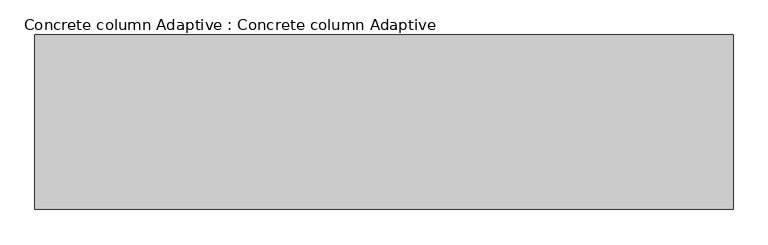
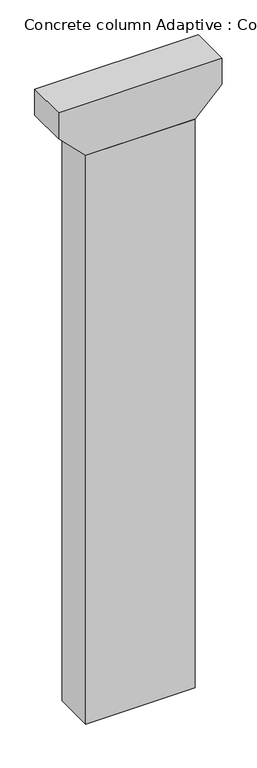
"""IFC4 building model written with IfcOpenShell, lengths in millimetres: proxy geometry, Concrete column Adaptive : Concrete column Adaptive."""

import ifcopenshell
import ifcopenshell.guid

model = None  # the IFC model being written
_history = None  # IfcOwnerHistory: only IFC2X3 demands one
_inside = {}  # id of a spatial element -> (the spatial element, [elements in it])
_under = {}  # id of a project, library or spatial element -> (it, [spatial elements below it])
_declared = {}  # id of a project -> (the project, [libraries it declares])
_typed = {}  # id of a type object -> (the type object, [elements of that type])
_made_of = {}  # id of a material, layer set ... -> (it, [elements and type objects made of it])


def new_model(schema):
    """Start an empty IFC model of exactly this schema.

    Asked for "IFC4X3", IfcOpenShell would pick the latest addendum, in which some entities
    have other attributes; the version numbers below select the first issue.
    IFC2X3 requires an IfcOwnerHistory on every rooted entity: one is made here for all.
    """
    global model, _history
    if schema == "IFC4X3":
        model = ifcopenshell.file(schema_version=(4, 3, 0, 0))
    else:
        model = ifcopenshell.file(schema=schema)
    _inside.clear()
    _under.clear()
    _declared.clear()
    _typed.clear()
    _made_of.clear()
    _history = None
    if model.schema == "IFC2X3":
        org = make("IfcOrganization", Name="unknown")
        user = make(
            "IfcPersonAndOrganization",
            ThePerson=make("IfcPerson", FamilyName="unknown"),
            TheOrganization=org,
        )
        app = make(
            "IfcApplication",
            ApplicationDeveloper=org,
            Version="unknown",
            ApplicationFullName="unknown",
            ApplicationIdentifier="unknown",
        )
        _history = make(
            "IfcOwnerHistory",
            OwningUser=user,
            OwningApplication=app,
            ChangeAction="ADDED",
            CreationDate=0,
        )
    return model


def make(cls, **values):
    """One entity of the class cls with the attributes given. An attribute that is None is left unset."""
    return model.create_entity(
        cls, **{name: value for name, value in values.items() if value is not None}
    )


def rooted(cls, **values):
    """An entity with a GlobalId (a new one), such as an element, a storey or a relation."""
    return make(cls, GlobalId=ifcopenshell.guid.new(), OwnerHistory=_history, **values)


def si_unit(unit_type, name, prefix=None):
    """IfcSIUnit, for example si_unit("LENGTHUNIT", "METRE", prefix="MILLI")."""
    return make("IfcSIUnit", UnitType=unit_type, Prefix=prefix, Name=name)


def assignment(units):
    """IfcUnitAssignment: the units of a project."""
    return None if units is None else make("IfcUnitAssignment", Units=units)


def point(xyz):
    """IfcCartesianPoint."""
    return None if xyz is None else make("IfcCartesianPoint", Coordinates=xyz)


def direction(xyz):
    """IfcDirection."""
    return None if xyz is None else make("IfcDirection", DirectionRatios=xyz)


def frame(location, z_axis=None, x_axis=None):
    """IfcAxis2Placement3D, a coordinate frame: its origin and axes. An axis left out is left unset."""
    return make(
        "IfcAxis2Placement3D",
        Location=point(location),
        Axis=direction(z_axis),
        RefDirection=direction(x_axis),
    )


def origin():
    """The frame at (0, 0, 0) with its axes left unset."""
    return frame((0.0, 0.0, 0.0))


def origin_with_axes():
    """The frame at (0, 0, 0) with the z axis (0, 0, 1) and the x axis (1, 0, 0) written out."""
    return frame((0.0, 0.0, 0.0), z_axis=(0.0, 0.0, 1.0), x_axis=(1.0, 0.0, 0.0))


def place(relative_to, where):
    """IfcLocalPlacement: puts the frame where relative to a parent placement (None: the world)."""
    return make(
        "IfcLocalPlacement", PlacementRelTo=relative_to, RelativePlacement=where
    )


def context(
    kind, dimensions, precision=None, world=None, true_north=None, identifier=None
):
    """IfcGeometricRepresentationContext, for example the 3D "Model" context."""
    return make(
        "IfcGeometricRepresentationContext",
        ContextIdentifier=identifier,
        ContextType=kind,
        CoordinateSpaceDimension=dimensions,
        Precision=precision,
        WorldCoordinateSystem=world,
        TrueNorth=true_north,
    )


def project(units=None, contexts=None):
    """IfcProject with its units and contexts."""
    return rooted(
        "IfcProject",
        Name="project",
        RepresentationContexts=contexts,
        UnitsInContext=assignment(units),
    )


def spatial(cls, under=None, at=None, **own):
    """A site, building, storey or space (cls), placed at a placement, below another one or the project."""
    s = rooted(cls, ObjectPlacement=at, **own)
    if under is not None:
        _under.setdefault(under.id(), (under, []))[1].append(s)
    return s


def polyline(points):
    """IfcPolyline through the points."""
    return make("IfcPolyline", Points=[point(p) for p in points])


def outline(outer, holes=None, kind="AREA"):
    """IfcArbitraryClosedProfileDef: a profile drawn as a closed curve; with holes, ...WithVoids."""
    if holes is None:
        return make("IfcArbitraryClosedProfileDef", ProfileType=kind, OuterCurve=outer)
    return make(
        "IfcArbitraryProfileDefWithVoids",
        ProfileType=kind,
        OuterCurve=outer,
        InnerCurves=holes,
    )


def extrude(swept, where, along, depth):
    """IfcExtrudedAreaSolid: the profile swept, set in the frame where, extruded along a direction by depth."""
    return make(
        "IfcExtrudedAreaSolid",
        SweptArea=swept,
        Position=where,
        ExtrudedDirection=direction(along),
        Depth=depth,
    )


def shape(context_of_items, identifier, shape_type, items):
    """IfcShapeRepresentation: the items that make up one representation, for example the "Body"."""
    return make(
        "IfcShapeRepresentation",
        ContextOfItems=context_of_items,
        RepresentationIdentifier=identifier,
        RepresentationType=shape_type,
        Items=items,
    )


def source(mapping_origin, context_of_items, identifier, shape_type, items):
    """IfcRepresentationMap: a shape defined once, which mapped items show again and again."""
    return make(
        "IfcRepresentationMap",
        MappingOrigin=mapping_origin,
        MappedRepresentation=shape(context_of_items, identifier, shape_type, items),
    )


def transform(
    local_origin,
    x_axis=None,
    y_axis=None,
    z_axis=None,
    scale=None,
    scale2=None,
    scale3=None,
    uniform=True,
):
    """IfcCartesianTransformationOperator3D, or its non-uniform kind. x_axis, y_axis, z_axis: its Axis1, 2, 3."""
    if uniform:
        return make(
            "IfcCartesianTransformationOperator3D",
            Axis1=direction(x_axis),
            Axis2=direction(y_axis),
            LocalOrigin=point(local_origin),
            Scale=scale,
            Axis3=direction(z_axis),
        )
    return make(
        "IfcCartesianTransformationOperator3DnonUniform",
        Axis1=direction(x_axis),
        Axis2=direction(y_axis),
        LocalOrigin=point(local_origin),
        Scale=scale,
        Axis3=direction(z_axis),
        Scale2=scale2,
        Scale3=scale3,
    )


def mapped(mapping_source, mapping_target):
    """IfcMappedItem: shows the shape of a source again, moved by a transform."""
    return make(
        "IfcMappedItem", MappingSource=mapping_source, MappingTarget=mapping_target
    )


def made_of(thing, what):
    """Note that an element or type object is made of a material, layer set ...; save() writes the relation."""
    if what is not None:
        _made_of.setdefault(what.id(), (what, []))[1].append(thing)
    return thing


def element(
    cls,
    number,
    at=None,
    inside=None,
    cuts=None,
    type_object=None,
    material=None,
    context=None,
    identifier="Body",
    shape_type=None,
    held_by="IfcProductDefinitionShape",
    body=None,
    shapes=None,
    **own,
):
    """One element of the class cls, such as IfcWall. Its Tag is "e" and its number.

    at: its placement. inside: the storey or other place that contains it. cuts: it is an
    opening in that element (IfcRelVoidsElement). A single representation is given by context,
    identifier, shape_type and body (its items); several are given by shapes. held_by: the class
    of the entity that holds the representations. save() writes the other relations.
    """
    e = rooted(cls, Tag="e%d" % number, ObjectPlacement=at, **own)
    if body is not None:
        shapes = [shape(context, identifier, shape_type, body)]
    if shapes is not None:
        e.Representation = make(held_by, Representations=shapes)
    if inside is not None:
        _inside.setdefault(inside.id(), (inside, []))[1].append(e)
    if cuts is not None:
        rooted(
            "IfcRelVoidsElement", RelatingBuildingElement=cuts, RelatedOpeningElement=e
        )
    if type_object is not None:
        _typed.setdefault(type_object.id(), (type_object, []))[1].append(e)
    return made_of(e, material)


def aggregate(whole, parts):
    """IfcRelAggregates: a whole, such as a stair, and the parts it consists of."""
    return rooted("IfcRelAggregates", RelatingObject=whole, RelatedObjects=parts)


def save(model, path):
    """Write the relations noted so far, then the file.

    IfcRelAggregates (storeys below a building ...), IfcRelContainedInSpatialStructure (elements
    in a storey), IfcRelDefinesByType, IfcRelAssociatesMaterial and IfcRelDeclares: one each for
    every whole, place, type object, material and project.
    """
    for whole, parts in _under.values():
        aggregate(whole, parts)
    for where, things in _inside.values():
        rooted(
            "IfcRelContainedInSpatialStructure",
            RelatedElements=things,
            RelatingStructure=where,
        )
    for kind, things in _typed.values():
        rooted("IfcRelDefinesByType", RelatedObjects=things, RelatingType=kind)
    for what, things in _made_of.values():
        rooted("IfcRelAssociatesMaterial", RelatedObjects=things, RelatingMaterial=what)
    for by, libraries in _declared.values():
        rooted("IfcRelDeclares", RelatingContext=by, RelatedDefinitions=libraries)
    model.write(path)


def concrete_column_adaptive_concrete_column_adaptive_2f6c8aee(model_context):
    return source(origin(), model_context, "Body", "SweptSolid", [
        extrude(outline(polyline([(48034.0, 6000.0), (48034.0, -6000.0), (46034.0, -6000.0), (44034.0, -4000.0), (44034.0, 4000.0), (46034.0, 6000.0), (48034.0, 6000.0)])), frame((0.0, -1500.0, 0.0), z_axis=(0.0, 1.0, 0.0), x_axis=(0.0, 0.0, 1.0)), (0.0, 0.0, 1.0), 3000.0),
        extrude(outline(polyline([(-4000.0, -1500.0), (-4000.0, 1500.0), (4000.0, 1500.0), (4000.0, -1500.0), (-4000.0, -1500.0)])), origin_with_axes(), (0.0, 0.0, 1.0), 44034.0),
    ])


if __name__ == "__main__":
    model = new_model("IFC4")
    model_context = context("Model", 3, world=origin())
    ifc_project = project(units=[si_unit("LENGTHUNIT", "METRE", prefix="MILLI")], contexts=[model_context])
    site = spatial("IfcSite", under=ifc_project)
    building = spatial("IfcBuilding", under=site)
    placement = place(None, origin())
    concrete_column_adaptive_concrete_column_adaptive_shape = concrete_column_adaptive_concrete_column_adaptive_2f6c8aee(model_context)
    element("IfcBuildingElementProxy", 1, Name="Concrete column Adaptive : Concrete column Adaptive", ObjectType="Concrete column Adaptive : Concrete column Adaptive", at=placement, inside=building, context=model_context, shape_type="MappedRepresentation", body=[
        mapped(concrete_column_adaptive_concrete_column_adaptive_shape, transform((0.0, 0.0, 0.0), x_axis=(1.0, 0.0, 0.0), y_axis=(0.0, 1.0, 0.0), z_axis=(0.0, 0.0, 1.0))),
    ])
    save(model, "model.ifc")

# Revit data of these elements
# Type "Concrete column Adaptive : Concrete column Adaptive"
#   Height [instance default] = 30000 mm
#   Default Elevation = 0
# Element 1 (IfcBuildingElementProxy, "Concrete column Adaptive : Concrete column Adaptive")
#   Height = 44034 mm
